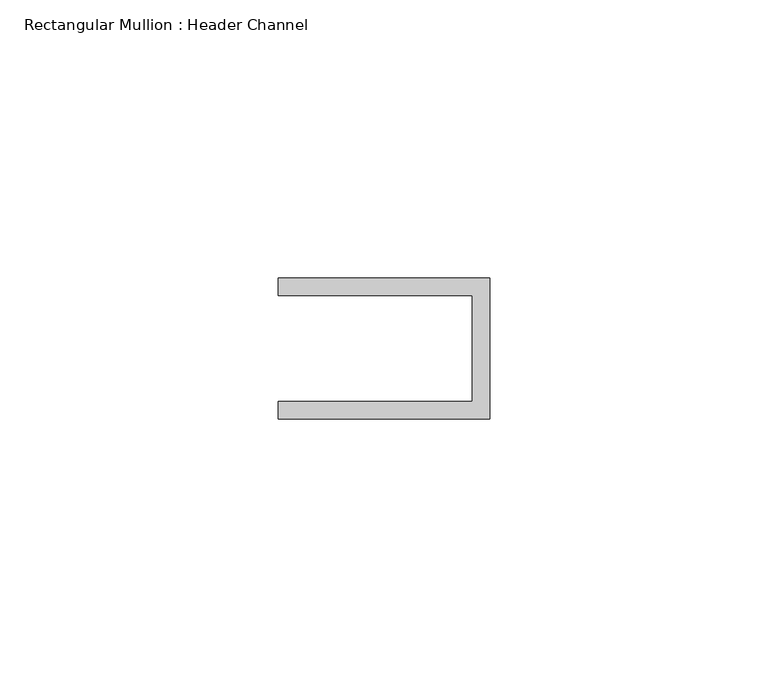
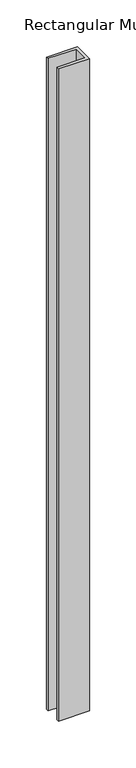
"""IFC4 building model written with IfcOpenShell, lengths in millimetres: member geometry, Rectangular Mullion : Header Channel."""

from ifc_helpers import new_model, si_unit, frame, origin, place, context, project, spatial, polyline, outline, extrude, source, transform, mapped, element, save


def rectangular_mullion_header_channel_6e33c34a(model_context):
    return source(origin(), model_context, "Body", "SweptSolid", [
        extrude(outline(polyline([(0.0, -12.7), (-38.1, -12.7), (-38.1, -9.525), (-3.175, -9.525), (-3.175, 9.525), (-38.1, 9.525), (-38.1, 12.7), (0.0, 12.7), (0.0, -12.7)])), frame((0.0, 0.0, -851.1267857), z_axis=(0.0, 0.0, 1.0), x_axis=(1.0, 0.0, 0.0)), (0.0, 0.0, 1.0), 851.1267857),
    ])


if __name__ == "__main__":
    model = new_model("IFC4")
    model_context = context("Model", 3, world=origin())
    ifc_project = project(units=[si_unit("LENGTHUNIT", "METRE", prefix="MILLI")], contexts=[model_context])
    site = spatial("IfcSite", under=ifc_project)
    building = spatial("IfcBuilding", under=site)
    placement = place(None, origin())
    rectangular_mullion_header_channel_shape = rectangular_mullion_header_channel_6e33c34a(model_context)
    element("IfcMember", 1, ObjectType="Rectangular Mullion : Header Channel", at=placement, inside=building, context=model_context, shape_type="MappedRepresentation", body=[
        mapped(rectangular_mullion_header_channel_shape, transform((0.0, 0.0, 0.0), x_axis=(1.0, 0.0, 0.0), y_axis=(0.0, 1.0, 0.0), z_axis=(0.0, 0.0, 1.0))),
    ])
    save(model, "model.ifc")

# Revit data of these elements
# Type "Rectangular Mullion : Header Channel"
#   built-in parameter 1007322 = 0.0833333 (stored number, unit not read)
#   built-in parameter 1007321 = -0.03125 (stored number, unit not read)
#   built-in parameter 1007320 = 0.0416667 (stored number, unit not read)
# Element 1 (IfcMember, "Rectangular Mullion : Header Channel")
#   Materials on its faces: "ALUM"
# Materials
#   "ALUM": class "Generic", colour RGB 157 157 157, transparency 0, Cost = 0
